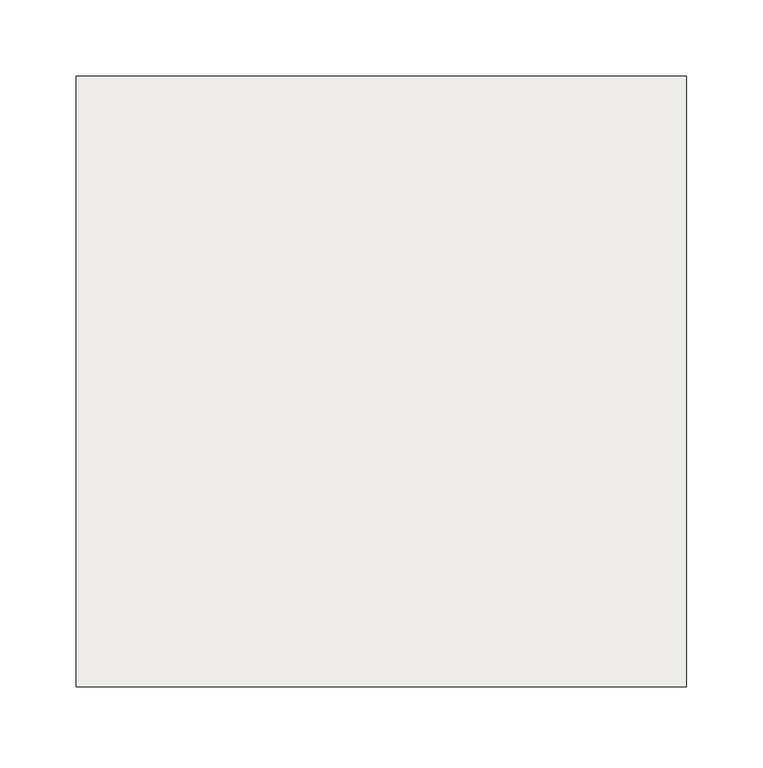
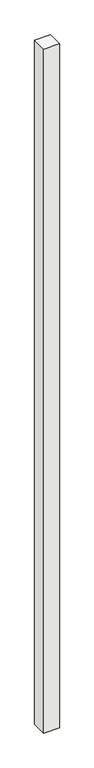
"""IFC4 building model written with IfcOpenShell, lengths in millimetres: footing geometry, NLRS_17_SFO_TLB_funderingspaal geheid beton prefab-AV-MMBPC_gen_rsf : heipaal beton prefab_gen__bxh 400x400."""

from ifc_helpers import new_model, si_unit, frame, origin, place, context, project, spatial, polyline, outline, extrude, source, transform, mapped, element, save


def footing_81e4ded3(model_context):
    return source(origin(), model_context, "Body", "SweptSolid", [
        extrude(outline(polyline([(200.0, -200.0), (-200.0, -200.0), (-200.0, 200.0), (200.0, 200.0), (200.0, -200.0)])), frame((0.0, 0.0, -20000.0), z_axis=(0.0, 0.0, 1.0), x_axis=(1.0, 0.0, 0.0)), (0.0, 0.0, 1.0), 18520.0),
    ])


if __name__ == "__main__":
    model = new_model("IFC4")
    model_context = context("Model", 3, world=origin())
    ifc_project = project(units=[si_unit("LENGTHUNIT", "METRE", prefix="MILLI")], contexts=[model_context])
    site = spatial("IfcSite", under=ifc_project)
    building = spatial("IfcBuilding", under=site)
    placement = place(None, origin())
    footing_shape = footing_81e4ded3(model_context)
    element("IfcFooting", 1, ObjectType="NLRS_17_SFO_TLB_funderingspaal geheid beton prefab-AV-MMBPC_gen_rsf : heipaal beton prefab_gen__bxh 400x400", at=placement, inside=building, context=model_context, shape_type="MappedRepresentation", body=[
        mapped(footing_shape, transform((0.0, 0.0, 0.0), x_axis=(1.0, 0.0, 0.0), y_axis=(0.0, 1.0, 0.0), z_axis=(0.0, 0.0, 1.0))),
    ])
    save(model, "model.ifc")

# Revit data of these elements
# Type "NLRS_17_SFO_TLB_funderingspaal geheid beton prefab-AV-MMBPC_gen_rsf : heipaal beton prefab_gen__bxh 400x400"
#   IfcExportAs = "IfcPile"
#   Type Comments = "prefab heipaal 400x400"
#   Model = " "
#   Manufacturer = " "
#   Description = "prefab heipaal 400x400"
#   Assembly Code = "17.21"
#   Width = 400 mm
#   Slanted Angle [instance default] = 0.00°
#   NLRS_S_draagvermogen_trek [instance default] = 0.00 kN
#   NLRS_S_draagvermogen_druk [instance default] = 0.00 kN
#   NLRS_C_lengte [instance default] = 1660 mm
#   NLRS_C_hoogte = 400 mm
#   NLRS_C_breedte = 400 mm
#   Height [instance default] = 1660 mm
#   Length [instance default] = 1660 mm
#   Angle [instance default] = 0.00°
#   Slanted [instance default] = 0
#   Structural Material = NLRS_f2_beton prefab_gen_rsf
#   Keynote = ""
# Element 1 (IfcFooting, "NLRS_17_SFO_TLB_funderingspaal geheid beton prefab-AV-MMBPC_gen_rsf : heipaal beton prefab_gen__bxh 400x400")
#   NLRS_C_lengte = 18520 mm
#   Height = 18520 mm
#   Length = 18520 mm
#   Materials on its faces: "NLRS_f2_beton prefab_gen_rsf"
# Materials
#   "NLRS_f2_beton prefab_gen_rsf": class "F - Niet gebakken kunststeen", colour RGB 129 133 118, transparency 0, Keynote = "f2", Manufacturer = "Revit Standards Foundation", URL = "www.revitstandards.org", Description = "beton prefab", Cost = 0
